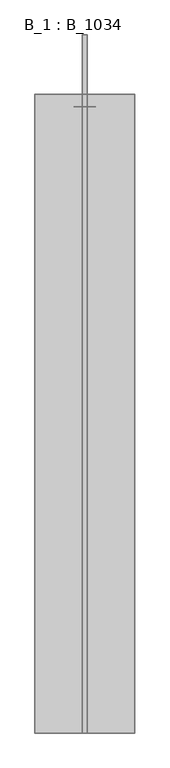
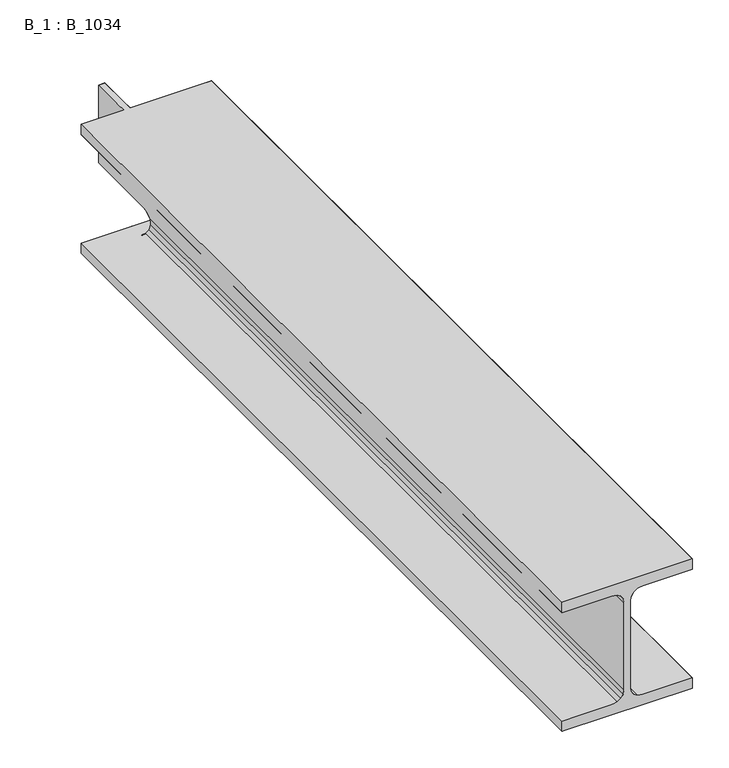
"""IFC4 building model written with IfcOpenShell, lengths in millimetres: beam geometry, B_1 : B_1034."""

from ifc_helpers import new_model, si_unit, origin, place, context, project, spatial, triangles, source, transform, mapped, element, save


def b_1_b_1034_869e73db(model_context):
    return source(origin(), model_context, "Body", "Tessellation", [
        triangles([(-25807.796814, -1443.0375, 15827.3750969), (-25807.796814, -1443.0375, 15809.9758682), (-25727.4063721, -1443.0375, 15809.9758682), (-25720.6998047, -1443.0375, 15808.641938), (-25715.0117798, -1443.0375, 15804.8427513), (-25711.2120117, -1443.0375, 15799.1570518), (-25709.8818604, -1443.0375, 15792.4499031), (-25709.8818604, -1443.0375, 15646.4000969), (-25711.2120117, -1443.0375, 15639.6929482), (-25715.0117798, -1443.0375, 15634.0072487), (-25720.6998047, -1443.0375, 15630.208062), (-25727.4063721, -1443.0375, 15628.8741318), (-25807.796814, -1443.0375, 15628.8741318), (-25807.796814, -1443.0375, 15611.4749031), (-25601.8047363, -1443.0375, 15611.4749031), (-25601.8047363, -1443.0375, 15628.8741318), (-25682.1951782, -1443.0375, 15628.8741318), (-25688.9017456, -1443.0375, 15630.208062), (-25694.5851196, -1443.0375, 15634.0072487), (-25698.3848877, -1443.0375, 15639.6929482), (-25699.7196899, -1443.0375, 15646.4000969), (-25699.7196899, -1443.0375, 15792.4499031), (-25698.3848877, -1443.0375, 15799.1570518), (-25694.5851196, -1443.0375, 15804.8427513), (-25688.9017456, -1443.0375, 15808.641938), (-25682.1951782, -1443.0375, 15809.9758682), (-25601.8047363, -1443.0375, 15809.9758682), (-25601.8047363, -1443.0375, 15827.3750969), (-25709.8818604, -4.7625, 15654.5280891), (-25709.8818604, -4.7625, 15784.3219109), (-25699.7196899, -4.7625, 15784.3219109), (-25699.7196899, -4.7625, 15654.5280891), (-25807.796814, -126.999997, 15809.9758682), (-25807.796814, -126.999997, 15827.3750969), (-25727.4063721, -126.999997, 15809.9758682), (-25715.0117798, -151.7576337, 15804.8427513), (-25720.6998047, -152.257803, 15808.641938), (-25711.2120117, -149.8813583, 15799.1570518), (-25713.8816162, -151.5345187, 15803.1480873), (-25709.8818604, -145.4888303, 15792.4499031), (-25710.7887817, -148.9970464, 15797.0220078), (-25709.8818604, -133.5740052, 15653.6624443), (-25709.8818604, -139.700003, 15651.1250992), (-25709.8818604, -144.9605104, 15647.088427), (-25709.8818604, -145.4888303, 15646.4000969), (-25709.8818604, -144.9605104, 15791.761573), (-25709.8818604, -139.700003, 15787.7249008), (-25709.8818604, -133.5740052, 15785.1875557), (-25709.8818604, -126.999997, 15784.3219109), (-25709.8818604, -126.999997, 15654.5280891), (-25711.2120117, -149.8813583, 15639.6929482), (-25710.7887817, -148.9970464, 15641.8279922), (-25715.0117798, -151.7576337, 15634.0072487), (-25713.8816162, -151.5345187, 15635.7019127), (-25720.6998047, -152.257803, 15630.208062), (-25807.796814, -126.999997, 15628.8741318), (-25727.4063721, -126.999997, 15628.8741318), (-25807.796814, -126.999997, 15611.4749031), (-25722.606665, -126.999997, 15611.4749031), (-25686.9948853, -126.999997, 15611.4749031), (-25601.8047363, -126.999997, 15611.4749031), (-25601.8047363, -126.999997, 15628.8741318), (-25682.1951782, -126.999997, 15628.8741318), (-25694.5851196, -151.7576337, 15634.0072487), (-25688.9017456, -152.257803, 15630.208062), (-25698.3848877, -149.8813583, 15639.6929482), (-25695.7199341, -151.5345187, 15635.7019127), (-25699.7196899, -145.4888303, 15646.4000969), (-25698.8127686, -148.9970464, 15641.8279922), (-25699.7196899, -139.700003, 15651.1250992), (-25699.7196899, -133.5740052, 15653.6624443), (-25699.7196899, -126.999997, 15654.5280891), (-25699.7196899, -126.999997, 15784.3219109), (-25699.7196899, -133.5740052, 15785.1875557), (-25699.7196899, -139.700003, 15787.7249008), (-25699.7196899, -144.9605104, 15791.761573), (-25699.7196899, -145.4888303, 15792.4499031), (-25699.7196899, -144.9605104, 15647.088427), (-25698.3848877, -149.8813583, 15799.1570518), (-25698.8127686, -148.9970464, 15797.0220078), (-25694.5851196, -151.7576337, 15804.8427513), (-25695.7199341, -151.5345187, 15803.1480873), (-25688.9017456, -152.257803, 15808.641938), (-25601.8047363, -126.999997, 15809.9758682), (-25682.1951782, -126.999997, 15809.9758682), (-25601.8047363, -126.999997, 15827.3750969), (-25686.9948853, -126.999997, 15827.3750969), (-25722.606665, -126.999997, 15827.3750969), (-25682.320752, -126.999997, 15809.9505791), (-25686.9948853, -126.999997, 15809.9505791), (-25722.606665, -126.999997, 15809.9505791), (-25727.2761475, -126.999997, 15809.9505791), (-25682.320752, -152.4, 15809.9505791), (-25727.2761475, -152.4, 15809.9505791), (-25683.469519, -152.4, 15809.7221046), (-25726.1273804, -152.4, 15809.7221046), (-25683.469519, -152.4, 15629.1278954), (-25726.1273804, -152.4, 15629.1278954), (-25727.2761475, -152.4, 15628.8994209), (-25682.320752, -152.4, 15628.8994209), (-25727.2761475, -126.999997, 15628.8994209), (-25682.320752, -126.999997, 15628.8994209), (-25686.9948853, -126.999997, 15628.8994209), (-25722.606665, -126.999997, 15628.8994209)], [[1, 2, 3], [26, 1, 3], [4, 5, 24], [6, 7, 22], [5, 6, 23], [25, 3, 4], [28, 26, 27], [28, 1, 26], [22, 23, 6], [24, 25, 4], [23, 24, 5], [3, 25, 26], [7, 21, 22], [9, 10, 20], [8, 9, 21], [13, 14, 12], [18, 11, 12], [12, 14, 17], [10, 11, 19], [20, 21, 9], [19, 20, 10], [18, 12, 17], [15, 16, 17], [14, 15, 17], [19, 11, 18], [8, 21, 7], [32, 29, 30], [30, 31, 32], [34, 33, 2], [2, 1, 34], [33, 35, 2], [3, 2, 35], [37, 36, 5], [5, 4, 37], [39, 38, 6], [36, 6, 5], [6, 36, 39], [41, 40, 7], [38, 7, 6], [7, 38, 41], [8, 7, 40], [8, 40, 45], [46, 44, 45], [48, 42, 43], [43, 44, 47], [40, 46, 45], [49, 42, 48], [48, 43, 47], [50, 49, 30], [50, 42, 49], [30, 29, 50], [47, 44, 46], [45, 52, 8], [51, 9, 8], [51, 8, 52], [51, 54, 9], [53, 10, 9], [53, 9, 54], [53, 55, 10], [11, 10, 55], [57, 56, 12], [13, 12, 56], [56, 58, 14], [14, 13, 56], [14, 58, 59], [14, 59, 15], [60, 61, 15], [60, 15, 59], [61, 62, 16], [16, 15, 61], [62, 63, 16], [17, 16, 63], [65, 64, 19], [19, 18, 65], [67, 66, 20], [64, 20, 19], [20, 64, 67], [69, 68, 21], [66, 21, 20], [21, 66, 69], [76, 77, 68], [70, 74, 75], [72, 32, 31], [72, 31, 73], [74, 71, 73], [75, 76, 78], [78, 76, 68], [78, 70, 75], [77, 21, 68], [72, 73, 71], [74, 70, 71], [77, 22, 21], [77, 80, 22], [79, 23, 22], [79, 22, 80], [79, 82, 23], [81, 24, 23], [81, 23, 82], [81, 83, 24], [25, 24, 83], [85, 84, 26], [27, 26, 84], [84, 86, 28], [28, 27, 84], [86, 87, 28], [88, 1, 28], [1, 88, 34], [88, 28, 87], [86, 85, 87], [85, 86, 84], [91, 88, 87], [34, 88, 35], [92, 35, 88], [34, 35, 33], [87, 85, 89], [89, 90, 87], [91, 87, 90], [88, 91, 92], [94, 92, 91], [94, 91, 93], [90, 89, 93], [90, 93, 91], [93, 95, 96], [96, 94, 93], [95, 83, 96], [81, 82, 36], [83, 81, 37], [39, 36, 82], [37, 96, 83], [36, 37, 81], [79, 80, 41], [82, 79, 39], [38, 39, 79], [41, 38, 79], [77, 76, 46], [80, 77, 41], [46, 40, 77], [40, 41, 77], [47, 46, 75], [76, 75, 46], [48, 47, 75], [75, 74, 48], [49, 48, 74], [74, 73, 49], [31, 30, 49], [49, 73, 31], [29, 32, 72], [72, 50, 29], [72, 71, 42], [42, 50, 72], [71, 70, 43], [43, 42, 71], [70, 78, 44], [44, 43, 70], [68, 69, 52], [78, 68, 44], [52, 45, 68], [45, 44, 68], [66, 67, 54], [69, 66, 52], [51, 52, 66], [54, 51, 66], [53, 54, 67], [98, 55, 97], [53, 64, 55], [67, 64, 53], [65, 97, 55], [64, 65, 55], [99, 98, 97], [97, 100, 99], [102, 103, 100], [104, 99, 100], [99, 104, 101], [104, 100, 103], [61, 60, 63], [63, 60, 102], [61, 63, 62], [102, 60, 103], [60, 104, 103], [59, 58, 57], [57, 58, 56], [59, 57, 101], [59, 101, 104], [59, 104, 60]], closed=False),
    ])


if __name__ == "__main__":
    model = new_model("IFC4")
    model_context = context("Model", 3, world=origin())
    ifc_project = project(units=[si_unit("LENGTHUNIT", "METRE", prefix="MILLI")], contexts=[model_context])
    site = spatial("IfcSite", under=ifc_project)
    building = spatial("IfcBuilding", under=site)
    placement = place(None, origin())
    b_1_b_1034_shape = b_1_b_1034_869e73db(model_context)
    element("IfcBeam", 1, ObjectType="B_1 : B_1034", at=placement, inside=building, context=model_context, shape_type="MappedRepresentation", body=[
        mapped(b_1_b_1034_shape, transform((0.0, 0.0, 0.0), x_axis=(1.0, 0.0, 0.0), y_axis=(0.0, 1.0, 0.0), z_axis=(0.0, 0.0, 1.0))),
    ])
    save(model, "model.ifc")

# Revit data of these elements
# Project information
#   IfcSite GUID = "oJcFLeXo4rgcjZ$xT65ur0"
#   IfcBuilding GUID = "hIkbrsvI41jdPtrPXtew81"
#   IfcProject GUID = "YUXJs3w44jVZO9Z8EqEW81"
#   NameOverride = "Job Site"
#   Project Issue Date = "Issue Date"
#   Project Status = "Project Status"
#   Client Name = "Owner"
#   Project Address = "Enter address here"
#   Project Name = "Project Name"
#   Project Number = "Project Number"
# Type "B_1 : B_1034"
#   IfcDescription = "W8x48"
#   NameOverride = "B_1034"
#   ObjectTypeOverride = "BEAM"
#   Cross_Section = "W8x48"
#   Material_Finish = "Red oxide"
#   Material_Grade = "A572-50"
#   Material_Piecemark = "e99"
#   Material_Type = "Wide Flange"
#   Member_Piecemark = "B_1034"
#   Member_Type = "BEAM"
#   Sequence = "TEST"
#   Zone = "5"
#   Actual_Ship_Date = "**NOT SET**"
#   Approval_Received_Date = "**NOT SET**"
#   Approval_Status = "Not reviewed"
#   Approval_Submitted_Date = "**NOT SET**"
#   Erected_Date = "**NOT SET**"
#   Fab_Completed_Date = "**NOT SET**"
#   Hold = "No"
#   Projected_Fab_Complete_Date = "**NOT SET**"
#   Projected_Ship_Date = "**NOT SET**"
#   Received_On_Site_Date = "**NOT SET**"
#   Released_For_Fab_Date = "**NOT SET**"
#   Revision = "No Revision"
